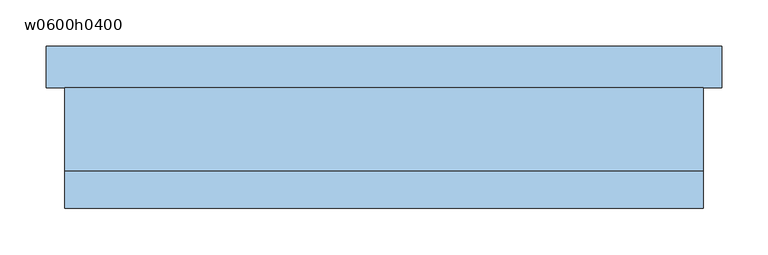
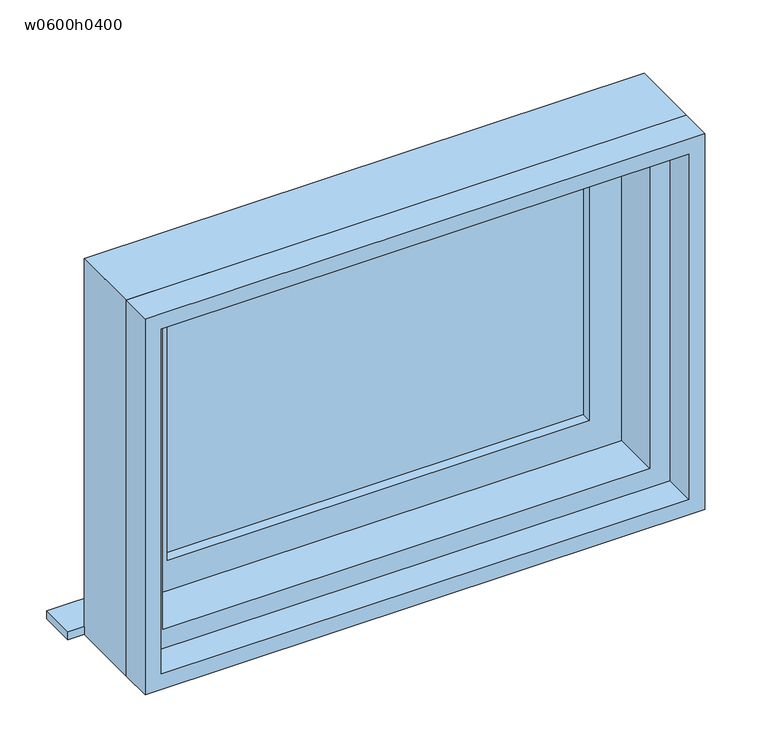
"""IFC4 building model written with IfcOpenShell, lengths in millimetres: window geometry, 横すべり窓 : w0600h0400."""

from ifc_helpers import new_model, si_unit, frame, origin, place, context, project, spatial, polyline, outline, extrude, source, transform, mapped, element, save


def w0600h0400_e5d73cd8(model_context):
    return source(origin(), model_context, "Body", "SweptSolid", [
        extrude(outline(polyline([(260.0, 27.5), (-260.0, 27.5), (-260.0, 32.5), (260.0, 32.5), (260.0, 27.5)])), frame((0.0, 0.0, 1640.0), z_axis=(0.0, 0.0, 1.0), x_axis=(1.0, 0.0, 0.0)), (0.0, 0.0, 1.0), 320.0),
        extrude(outline(polyline([(2000.0, 300.0), (2000.0, -300.0), (1600.0, -300.0), (1600.0, 300.0), (2000.0, 300.0)]), holes=[polyline([(1960.0, -260.0), (1960.0, 260.0), (1640.0, 260.0), (1640.0, -260.0), (1960.0, -260.0)])]), frame((0.0, 15.0, 0.0), z_axis=(0.0, 1.0, 0.0), x_axis=(0.0, 0.0, 1.0)), (0.0, 0.0, 1.0), 30.0),
        extrude(outline(polyline([(365.0, 90.0), (365.0, 45.0), (-365.0, 45.0), (-365.0, 90.0), (365.0, 90.0)])), frame((0.0, 0.0, 1555.0), z_axis=(0.0, 0.0, 1.0), x_axis=(1.0, 0.0, 0.0)), (0.0, 0.0, 1.0), 10.0),
        extrude(outline(polyline([(2045.0, 345.0), (2045.0, -345.0), (1555.0, -345.0), (1555.0, 345.0), (2045.0, 345.0)]), holes=[polyline([(1575.0, -325.0), (2025.0, -325.0), (2025.0, 325.0), (1575.0, 325.0), (1575.0, -325.0)])]), frame((0.0, -85.0, 0.0), z_axis=(0.0, 1.0, 0.0), x_axis=(0.0, 0.0, 1.0)), (0.0, 0.0, 1.0), 40.0),
        extrude(outline(polyline([(2045.0, -345.0), (1555.0, -345.0), (1555.0, 345.0), (2045.0, 345.0), (2045.0, -345.0)]), holes=[polyline([(2000.0, 300.0), (1600.0, 300.0), (1600.0, -300.0), (2000.0, -300.0), (2000.0, 300.0)])]), frame((0.0, -45.0, 0.0), z_axis=(0.0, 1.0, 0.0), x_axis=(0.0, 0.0, 1.0)), (0.0, 0.0, 1.0), 90.0),
    ])


if __name__ == "__main__":
    model = new_model("IFC4")
    model_context = context("Model", 3, world=origin())
    ifc_project = project(units=[si_unit("LENGTHUNIT", "METRE", prefix="MILLI")], contexts=[model_context])
    site = spatial("IfcSite", under=ifc_project)
    building = spatial("IfcBuilding", under=site)
    placement = place(None, origin())
    w0600h0400_shape = w0600h0400_e5d73cd8(model_context)
    element("IfcWindow", 1, ObjectType="横すべり窓 : w0600h0400", at=placement, inside=building, context=model_context, shape_type="MappedRepresentation", body=[
        mapped(w0600h0400_shape, transform((0.0, 0.0, 0.0), x_axis=(1.0, 0.0, 0.0), y_axis=(0.0, 1.0, 0.0), z_axis=(0.0, 0.0, 1.0))),
    ])
    save(model, "model.ifc")

# Revit data of these elements
# Type "横すべり窓 : w0600h0400"
#   Construction Type Id = "GSP4R"
#   Analytic Construction = "1/8 インチ ピルキントン一重ガラス"
#   Type Mark = "76"
#   Operation = "シングルパネル"
#   Keynote = "08520.S1"
#   Visual Light Transmittance = 0.9
#   Solar Heat Gain Coefficient = 0.86
#   Heat Transfer Coefficient (U) = 6.7069 W/(m²·K)
#   Height = 400 mm
#   既定の腰高 = 1600 mm
#   Width = 600 mm
#   額縁見附 = 20 mm
#   額縁ちり = 10 mm
#   サッシ見附 = 45 mm
#   サッシの幅 = 90 mm
#   サッシ額縁 [instance default] = none
#   サッシ本体 [instance default] = none
#   サッシガラス [instance default] = ガラス - 透明
#   Wall Closure = (empty or 0)
#   Type Comments = ""
#   Assembly Code = ""
# Element 1 (IfcWindow, "横すべり窓 : w0600h0400")
#   Materials on its faces: "ガラス - 透明"
# Materials
#   "ガラス - 透明": class "ガラス", colour RGB 0 128 192, transparency 0.9, Cost = 0
